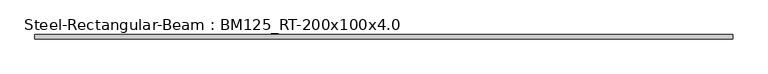
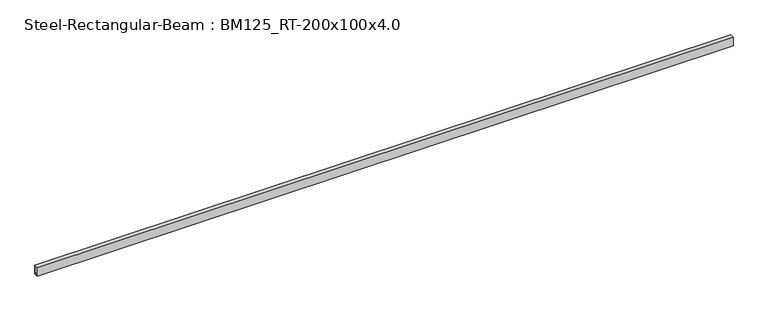
"""IFC4 building model written with IfcOpenShell, lengths in millimetres: beam geometry, Steel-Rectangular-Beam : BM125_RT-200x100x4.0."""

from ifc_helpers import new_model, si_unit, frame, origin, place, context, project, spatial, polyline, outline, extrude, source, transform, mapped, element, save


def steel_rectangular_beam_bm125_rt_200x100x4_0_52f716dd(model_context):
    return source(origin(), model_context, "Body", "SweptSolid", [
        extrude(outline(polyline([(-50.0, 100.0), (50.0, 100.0), (50.0, -100.0), (-50.0, -100.0), (-50.0, 100.0)]), holes=[polyline([(46.0, -96.0), (46.0, 96.0), (-46.0, 96.0), (-46.0, -96.0), (46.0, -96.0)])]), frame((-8000.0, 0.0, 0.0), z_axis=(1.0, 0.0, 0.0), x_axis=(0.0, 1.0, 0.0)), (0.0, 0.0, 1.0), 16000.0),
        extrude(outline(polyline([(-50.0, 100.0), (50.0, 100.0), (50.0, -100.0), (-50.0, -100.0), (-50.0, 100.0)]), holes=[polyline([(46.0, -96.0), (46.0, 96.0), (-46.0, 96.0), (-46.0, -96.0), (46.0, -96.0)])]), frame((-8000.0, 0.0, 0.0), z_axis=(1.0, 0.0, 0.0), x_axis=(0.0, 1.0, 0.0)), (0.0, 0.0, 1.0), 16000.0),
        extrude(outline(polyline([(-50.0, 100.0), (50.0, 100.0), (50.0, -100.0), (-50.0, -100.0), (-50.0, 100.0)]), holes=[polyline([(46.0, -96.0), (46.0, 96.0), (-46.0, 96.0), (-46.0, -96.0), (46.0, -96.0)])]), frame((-8000.0, 0.0, 0.0), z_axis=(1.0, 0.0, 0.0), x_axis=(0.0, 1.0, 0.0)), (0.0, 0.0, 1.0), 16000.0),
        extrude(outline(polyline([(-50.0, 100.0), (50.0, 100.0), (50.0, -100.0), (-50.0, -100.0), (-50.0, 100.0)]), holes=[polyline([(46.0, -96.0), (46.0, 96.0), (-46.0, 96.0), (-46.0, -96.0), (46.0, -96.0)])]), frame((-8000.0, 0.0, 0.0), z_axis=(1.0, 0.0, 0.0), x_axis=(0.0, 1.0, 0.0)), (0.0, 0.0, 1.0), 16000.0),
    ])


if __name__ == "__main__":
    model = new_model("IFC4")
    model_context = context("Model", 3, world=origin())
    ifc_project = project(units=[si_unit("LENGTHUNIT", "METRE", prefix="MILLI")], contexts=[model_context])
    site = spatial("IfcSite", under=ifc_project)
    building = spatial("IfcBuilding", under=site)
    placement = place(None, origin())
    steel_rectangular_beam_bm125_rt_200x100x4_0_shape = steel_rectangular_beam_bm125_rt_200x100x4_0_52f716dd(model_context)
    element("IfcBeam", 1, ObjectType="Steel-Rectangular-Beam : BM125_RT-200x100x4.0", at=placement, inside=building, context=model_context, shape_type="MappedRepresentation", body=[
        mapped(steel_rectangular_beam_bm125_rt_200x100x4_0_shape, transform((0.0, 0.0, 0.0), x_axis=(1.0, 0.0, 0.0), y_axis=(0.0, 1.0, 0.0), z_axis=(0.0, 0.0, 1.0))),
    ])
    save(model, "model.ifc")

# Revit data of these elements
# Type "Steel-Rectangular-Beam : BM125_RT-200x100x4.0"
#   t = 4 mm
#   Mass per Unit Length = 18.35 kg/m
#   Surface Area = 0.60 m²/m
#   Sectional Area = 1856.0 cm²
#   Length [instance default] = 3000 mm
#   H = 200 mm
#   B = 100 mm
#   hec_material4 [instance default] = none
#   hec_material3 [instance default] = none
#   hec_material2 [instance default] = none
#   hec_material1 [instance default] = none
#   Structural Material [instance default] = none
# Element 1 (IfcBeam, "Steel-Rectangular-Beam : BM125_RT-200x100x4.0")
#   hec_material2 = S01AA010-00001_Main Steel Structure Fabrication Work_Shelter/Building_Steel Painting/Coating_for Non-Fireproofed Steel Surface, Surface Preparation, Primer, Second & Final Coat
#   hec_material1 = S03AA007-00001_Main Steel Structure Erection Work_Girth & Purlin
#   Structural Material = S01AA007-00001_Main Steel Structure Fabrication Work_Shelter/Building_Girth & Purlin
#   Materials on its faces: "S01AA010-00001_Main Steel Structure Fabrication Work_Shelter/Building_Steel Painting/Coating_for Non-Fireproofed Steel Surface, Surface Preparation, Primer, Second & Final Coat"
# Materials
#   "S01AA010-00001_Main Steel Structure Fabrication Work_Shelter/Building_Steel Painting/Coating_for Non-Fireproofed Steel Surface, Surface Preparation, Primer, Second & Final Coat": class "Metal", colour RGB 120 120 120, transparency 0, Description = "Paint finished steel", W00) Work Master Code = "S01AA010-00001", W01) Work Master_Lv1 = "Main Steel Structure Fabrication Work", W02) Work Master_Lv2 = "Shelter/Building", W03) Work Master_Spec.1 = "Steel Painting/Coating", W04) Work Master_Spec.2 = "for Non-Fireproofed Steel Surface, Surface Preparation, Primer, Second & Final Coat", Cost = 0
#   "S03AA007-00001_Main Steel Structure Erection Work_Girth & Purlin": class "Metal", colour RGB 120 120 120, transparency 0, Comments = "(30KG/M>Weight)", Description = "Structural steel 50ksi", W00) Work Master Code = "S03AA007-00001", W01) Work Master_Lv1 = "Main Steel Structure Erection Work", W02) Work Master_Lv2 = "Shelter/Building", W03) Work Master_Spec.1 = "Girth & Purlin", Cost = 0
#   "S01AA007-00001_Main Steel Structure Fabrication Work_Shelter/Building_Girth & Purlin": class "Metal", colour RGB 120 120 120, transparency 0, Comments = "(30KG/M>Weight)", Description = "Structural steel 50ksi", W00) Work Master Code = "S01AA007-00001", W01) Work Master_Lv1 = "Main Steel Structure Fabrication Work", W02) Work Master_Lv2 = "Shelter/Building", W03) Work Master_Spec.1 = "Girth & Purlin", Cost = 0
